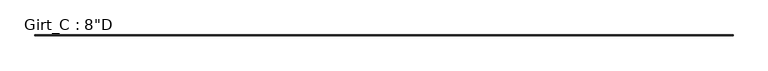
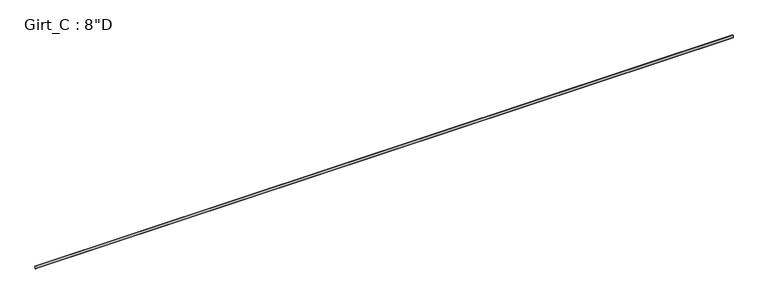
"""IFC4 building model written with IfcOpenShell, lengths in millimetres: beam geometry."""

from ifc_helpers import new_model, si_unit, point, frame, frame_2d, origin, place, context, project, spatial, polyline, circle_curve, trimmed, segment, composite_curve, outline, extrude, source, transform, mapped, element, save


def beam_b3f4e8ac(model_context):
    return source(origin(), model_context, "Body", "SweptSolid", [
        extrude(outline(composite_curve([segment(polyline([(63.5, 101.6), (75.745104, 87.0068534), (73.6169367, 85.221109), (62.204539, 98.821875), (3.3005807, 98.821875)]), True, "CONTINUOUS"), segment(trimmed(circle_curve(frame_2d((3.3741066, 96.8381931)), 1.9850441), [point((3.3005807, 98.821875))], [point((1.3890625, 96.8381931))], True, "CARTESIAN"), True, "CONTINUOUS"), segment(polyline([(1.3890625, 96.8381931), (1.3890625, -96.8389339)]), True, "CONTINUOUS"), segment(trimmed(circle_curve(frame_2d((3.3748024, -96.8389339)), 1.9857399), [point((1.3890625, -96.8389339))], [point((3.2694106, -98.821875))], True, "CARTESIAN"), True, "CONTINUOUS"), segment(polyline([(3.2694106, -98.821875), (62.204539, -98.821875), (73.6169367, -85.221109), (75.745104, -87.0068534), (63.5, -101.6), (3.3734375, -101.6)]), True, "CONTINUOUS"), segment(trimmed(circle_curve(frame_2d((3.3734375, -96.8375)), 4.7625), [point((3.3734375, -101.6))], [point((-1.3890625, -96.8375))], False, "CARTESIAN"), True, "CONTINUOUS"), segment(polyline([(-1.3890625, -96.8375), (-1.3890625, 96.8375)]), True, "CONTINUOUS"), segment(trimmed(circle_curve(frame_2d((3.3734375, 96.8375)), 4.7625), [point((-1.3890625, 96.8375))], [point((3.3734375, 101.6))], False, "CARTESIAN"), True, "CONTINUOUS"), segment(polyline([(3.3734375, 101.6), (63.5, 101.6)]), True, "CONTINUOUS")], self_intersect=False)), frame((-31019.75, 0.0, 0.0), z_axis=(1.0, 0.0, 0.0), x_axis=(0.0, 1.0, 0.0)), (0.0, 0.0, 1.0), 62236.35),
    ])


if __name__ == "__main__":
    model = new_model("IFC4")
    model_context = context("Model", 3, world=origin())
    ifc_project = project(units=[si_unit("LENGTHUNIT", "METRE", prefix="MILLI")], contexts=[model_context])
    site = spatial("IfcSite", under=ifc_project)
    building = spatial("IfcBuilding", under=site)
    placement = place(None, origin())
    beam_shape = beam_b3f4e8ac(model_context)
    element("IfcBeam", 1, ObjectType="Girt_C : 8\"D", at=placement, inside=building, context=model_context, shape_type="MappedRepresentation", body=[
        mapped(beam_shape, transform((0.0, 0.0, 0.0), x_axis=(1.0, 0.0, 0.0), y_axis=(0.0, 1.0, 0.0), z_axis=(0.0, 0.0, 1.0))),
    ])
    save(model, "model.ifc")

# Revit data of these elements
# Type "Girt_C : 8\"D"
#   Web_Thickness = 0' - 0 7/64"
#   Length [instance default] = 10' - 0"
#   Leg_1 = 0' - 2 1/2"
#   Height = 0' - 8"
#   Structural Material [instance default] = none
# Element 1 (IfcBeam, "Girt_C : 8\"D")
#   Structural Material = Steel
#   Materials on its faces: "Steel"
# Materials
#   "Steel": class "Metal", colour RGB 118 118 114, transparency 0, Description = "Steel, mill finish", Cost = 0
